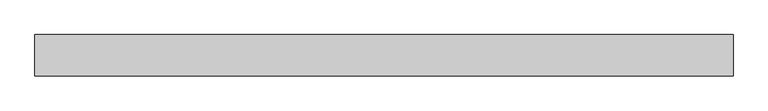
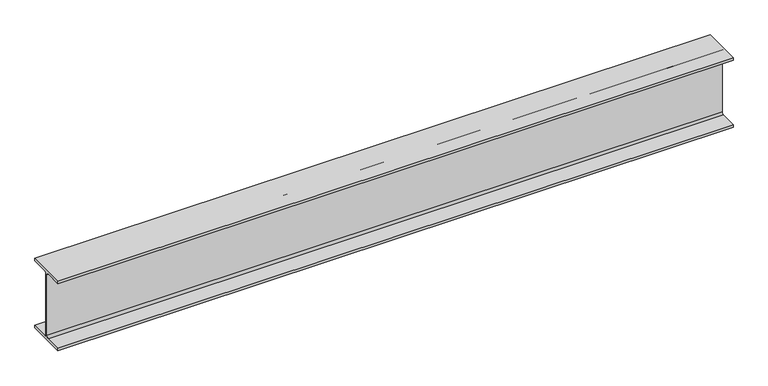
"""IFC4 building model written with IfcOpenShell, lengths in millimetres: beam geometry, Old_Steel Beam_H-KSD3502 : H_SB_ASB_H-250×125x6x9."""

import ifcopenshell
import ifcopenshell.guid

model = None  # the IFC model being written
_history = None  # IfcOwnerHistory: only IFC2X3 demands one
_inside = {}  # id of a spatial element -> (the spatial element, [elements in it])
_under = {}  # id of a project, library or spatial element -> (it, [spatial elements below it])
_declared = {}  # id of a project -> (the project, [libraries it declares])
_typed = {}  # id of a type object -> (the type object, [elements of that type])
_made_of = {}  # id of a material, layer set ... -> (it, [elements and type objects made of it])


def new_model(schema):
    """Start an empty IFC model of exactly this schema.

    Asked for "IFC4X3", IfcOpenShell would pick the latest addendum, in which some entities
    have other attributes; the version numbers below select the first issue.
    IFC2X3 requires an IfcOwnerHistory on every rooted entity: one is made here for all.
    """
    global model, _history
    if schema == "IFC4X3":
        model = ifcopenshell.file(schema_version=(4, 3, 0, 0))
    else:
        model = ifcopenshell.file(schema=schema)
    _inside.clear()
    _under.clear()
    _declared.clear()
    _typed.clear()
    _made_of.clear()
    _history = None
    if model.schema == "IFC2X3":
        org = make("IfcOrganization", Name="unknown")
        user = make(
            "IfcPersonAndOrganization",
            ThePerson=make("IfcPerson", FamilyName="unknown"),
            TheOrganization=org,
        )
        app = make(
            "IfcApplication",
            ApplicationDeveloper=org,
            Version="unknown",
            ApplicationFullName="unknown",
            ApplicationIdentifier="unknown",
        )
        _history = make(
            "IfcOwnerHistory",
            OwningUser=user,
            OwningApplication=app,
            ChangeAction="ADDED",
            CreationDate=0,
        )
    return model


def make(cls, **values):
    """One entity of the class cls with the attributes given. An attribute that is None is left unset."""
    return model.create_entity(
        cls, **{name: value for name, value in values.items() if value is not None}
    )


def rooted(cls, **values):
    """An entity with a GlobalId (a new one), such as an element, a storey or a relation."""
    return make(cls, GlobalId=ifcopenshell.guid.new(), OwnerHistory=_history, **values)


def si_unit(unit_type, name, prefix=None):
    """IfcSIUnit, for example si_unit("LENGTHUNIT", "METRE", prefix="MILLI")."""
    return make("IfcSIUnit", UnitType=unit_type, Prefix=prefix, Name=name)


def assignment(units):
    """IfcUnitAssignment: the units of a project."""
    return None if units is None else make("IfcUnitAssignment", Units=units)


def point(xyz):
    """IfcCartesianPoint."""
    return None if xyz is None else make("IfcCartesianPoint", Coordinates=xyz)


def direction(xyz):
    """IfcDirection."""
    return None if xyz is None else make("IfcDirection", DirectionRatios=xyz)


def frame(location, z_axis=None, x_axis=None):
    """IfcAxis2Placement3D, a coordinate frame: its origin and axes. An axis left out is left unset."""
    return make(
        "IfcAxis2Placement3D",
        Location=point(location),
        Axis=direction(z_axis),
        RefDirection=direction(x_axis),
    )


def frame_2d(location, x_axis=None):
    """IfcAxis2Placement2D, a coordinate frame in the plane: its origin and x axis."""
    return make(
        "IfcAxis2Placement2D", Location=point(location), RefDirection=direction(x_axis)
    )


def origin():
    """The frame at (0, 0, 0) with its axes left unset."""
    return frame((0.0, 0.0, 0.0))


def place(relative_to, where):
    """IfcLocalPlacement: puts the frame where relative to a parent placement (None: the world)."""
    return make(
        "IfcLocalPlacement", PlacementRelTo=relative_to, RelativePlacement=where
    )


def context(
    kind, dimensions, precision=None, world=None, true_north=None, identifier=None
):
    """IfcGeometricRepresentationContext, for example the 3D "Model" context."""
    return make(
        "IfcGeometricRepresentationContext",
        ContextIdentifier=identifier,
        ContextType=kind,
        CoordinateSpaceDimension=dimensions,
        Precision=precision,
        WorldCoordinateSystem=world,
        TrueNorth=true_north,
    )


def project(units=None, contexts=None):
    """IfcProject with its units and contexts."""
    return rooted(
        "IfcProject",
        Name="project",
        RepresentationContexts=contexts,
        UnitsInContext=assignment(units),
    )


def spatial(cls, under=None, at=None, **own):
    """A site, building, storey or space (cls), placed at a placement, below another one or the project."""
    s = rooted(cls, ObjectPlacement=at, **own)
    if under is not None:
        _under.setdefault(under.id(), (under, []))[1].append(s)
    return s


def polyline(points):
    """IfcPolyline through the points."""
    return make("IfcPolyline", Points=[point(p) for p in points])


def circle_curve(where, radius):
    """IfcCircle in the frame where."""
    return make("IfcCircle", Position=where, Radius=radius)


def trimmed(basis, trim1, trim2, sense, master):
    """IfcTrimmedCurve: the piece of a basis curve between two trims."""
    return make(
        "IfcTrimmedCurve",
        BasisCurve=basis,
        Trim1=trim1,
        Trim2=trim2,
        SenseAgreement=sense,
        MasterRepresentation=master,
    )


def segment(curve, same_sense, transition):
    """IfcCompositeCurveSegment."""
    return make(
        "IfcCompositeCurveSegment",
        Transition=transition,
        SameSense=same_sense,
        ParentCurve=curve,
    )


def composite_curve(segments, self_intersect=None):
    """IfcCompositeCurve: segments joined end to end."""
    return make("IfcCompositeCurve", Segments=segments, SelfIntersect=self_intersect)


def outline(outer, holes=None, kind="AREA"):
    """IfcArbitraryClosedProfileDef: a profile drawn as a closed curve; with holes, ...WithVoids."""
    if holes is None:
        return make("IfcArbitraryClosedProfileDef", ProfileType=kind, OuterCurve=outer)
    return make(
        "IfcArbitraryProfileDefWithVoids",
        ProfileType=kind,
        OuterCurve=outer,
        InnerCurves=holes,
    )


def extrude(swept, where, along, depth):
    """IfcExtrudedAreaSolid: the profile swept, set in the frame where, extruded along a direction by depth."""
    return make(
        "IfcExtrudedAreaSolid",
        SweptArea=swept,
        Position=where,
        ExtrudedDirection=direction(along),
        Depth=depth,
    )


def shape(context_of_items, identifier, shape_type, items):
    """IfcShapeRepresentation: the items that make up one representation, for example the "Body"."""
    return make(
        "IfcShapeRepresentation",
        ContextOfItems=context_of_items,
        RepresentationIdentifier=identifier,
        RepresentationType=shape_type,
        Items=items,
    )


def source(mapping_origin, context_of_items, identifier, shape_type, items):
    """IfcRepresentationMap: a shape defined once, which mapped items show again and again."""
    return make(
        "IfcRepresentationMap",
        MappingOrigin=mapping_origin,
        MappedRepresentation=shape(context_of_items, identifier, shape_type, items),
    )


def transform(
    local_origin,
    x_axis=None,
    y_axis=None,
    z_axis=None,
    scale=None,
    scale2=None,
    scale3=None,
    uniform=True,
):
    """IfcCartesianTransformationOperator3D, or its non-uniform kind. x_axis, y_axis, z_axis: its Axis1, 2, 3."""
    if uniform:
        return make(
            "IfcCartesianTransformationOperator3D",
            Axis1=direction(x_axis),
            Axis2=direction(y_axis),
            LocalOrigin=point(local_origin),
            Scale=scale,
            Axis3=direction(z_axis),
        )
    return make(
        "IfcCartesianTransformationOperator3DnonUniform",
        Axis1=direction(x_axis),
        Axis2=direction(y_axis),
        LocalOrigin=point(local_origin),
        Scale=scale,
        Axis3=direction(z_axis),
        Scale2=scale2,
        Scale3=scale3,
    )


def mapped(mapping_source, mapping_target):
    """IfcMappedItem: shows the shape of a source again, moved by a transform."""
    return make(
        "IfcMappedItem", MappingSource=mapping_source, MappingTarget=mapping_target
    )


def made_of(thing, what):
    """Note that an element or type object is made of a material, layer set ...; save() writes the relation."""
    if what is not None:
        _made_of.setdefault(what.id(), (what, []))[1].append(thing)
    return thing


def element(
    cls,
    number,
    at=None,
    inside=None,
    cuts=None,
    type_object=None,
    material=None,
    context=None,
    identifier="Body",
    shape_type=None,
    held_by="IfcProductDefinitionShape",
    body=None,
    shapes=None,
    **own,
):
    """One element of the class cls, such as IfcWall. Its Tag is "e" and its number.

    at: its placement. inside: the storey or other place that contains it. cuts: it is an
    opening in that element (IfcRelVoidsElement). A single representation is given by context,
    identifier, shape_type and body (its items); several are given by shapes. held_by: the class
    of the entity that holds the representations. save() writes the other relations.
    """
    e = rooted(cls, Tag="e%d" % number, ObjectPlacement=at, **own)
    if body is not None:
        shapes = [shape(context, identifier, shape_type, body)]
    if shapes is not None:
        e.Representation = make(held_by, Representations=shapes)
    if inside is not None:
        _inside.setdefault(inside.id(), (inside, []))[1].append(e)
    if cuts is not None:
        rooted(
            "IfcRelVoidsElement", RelatingBuildingElement=cuts, RelatedOpeningElement=e
        )
    if type_object is not None:
        _typed.setdefault(type_object.id(), (type_object, []))[1].append(e)
    return made_of(e, material)


def aggregate(whole, parts):
    """IfcRelAggregates: a whole, such as a stair, and the parts it consists of."""
    return rooted("IfcRelAggregates", RelatingObject=whole, RelatedObjects=parts)


def save(model, path):
    """Write the relations noted so far, then the file.

    IfcRelAggregates (storeys below a building ...), IfcRelContainedInSpatialStructure (elements
    in a storey), IfcRelDefinesByType, IfcRelAssociatesMaterial and IfcRelDeclares: one each for
    every whole, place, type object, material and project.
    """
    for whole, parts in _under.values():
        aggregate(whole, parts)
    for where, things in _inside.values():
        rooted(
            "IfcRelContainedInSpatialStructure",
            RelatedElements=things,
            RelatingStructure=where,
        )
    for kind, things in _typed.values():
        rooted("IfcRelDefinesByType", RelatedObjects=things, RelatingType=kind)
    for what, things in _made_of.values():
        rooted("IfcRelAssociatesMaterial", RelatedObjects=things, RelatingMaterial=what)
    for by, libraries in _declared.values():
        rooted("IfcRelDeclares", RelatingContext=by, RelatedDefinitions=libraries)
    model.write(path)


def beam_b824a9ea(model_context):
    return source(origin(), model_context, "Body", "SweptSolid", [
        extrude(outline(composite_curve([segment(polyline([(82.5, -141.5), (82.5, -151.7), (-82.5, -151.7), (-82.5, -141.5), (-11.9, -141.5)]), True, "CONTINUOUS"), segment(trimmed(circle_curve(frame_2d((-11.9, -132.6)), 8.9), [point((-11.9, -141.5))], [point((-3.0, -132.6))], True, "CARTESIAN"), True, "CONTINUOUS"), segment(polyline([(-3.0, -132.6), (-3.0, 132.6)]), True, "CONTINUOUS"), segment(trimmed(circle_curve(frame_2d((-11.9, 132.6)), 8.9), [point((-3.0, 132.6))], [point((-11.9, 141.5))], True, "CARTESIAN"), True, "CONTINUOUS"), segment(polyline([(-11.9, 141.5), (-82.5, 141.5), (-82.5, 151.7), (82.5, 151.7), (82.5, 141.5), (11.9, 141.5)]), True, "CONTINUOUS"), segment(trimmed(circle_curve(frame_2d((11.9, 132.6)), 8.9), [point((11.9, 141.5))], [point((3.0, 132.6))], True, "CARTESIAN"), True, "CONTINUOUS"), segment(polyline([(3.0, 132.6), (3.0, -132.6)]), True, "CONTINUOUS"), segment(trimmed(circle_curve(frame_2d((11.9, -132.6)), 8.9), [point((3.0, -132.6))], [point((11.9, -141.5))], True, "CARTESIAN"), True, "CONTINUOUS"), segment(polyline([(11.9, -141.5), (82.5, -141.5)]), True, "CONTINUOUS")], self_intersect=False)), frame((-1382.2982577, 0.0, 0.0), z_axis=(1.0, 0.0, 0.0), x_axis=(0.0, 1.0, 0.0)), (0.0, 0.0, 1.0), 2794.5982507),
    ])


if __name__ == "__main__":
    model = new_model("IFC4")
    model_context = context("Model", 3, world=origin())
    ifc_project = project(units=[si_unit("LENGTHUNIT", "METRE", prefix="MILLI")], contexts=[model_context])
    site = spatial("IfcSite", under=ifc_project)
    building = spatial("IfcBuilding", under=site)
    placement = place(None, origin())
    beam_shape = beam_b824a9ea(model_context)
    element("IfcBeam", 1, ObjectType="Old_Steel Beam_H-KSD3502 : H_SB_ASB_H-250×125x6x9", at=placement, inside=building, context=model_context, shape_type="MappedRepresentation", body=[
        mapped(beam_shape, transform((0.0, 0.0, 0.0), x_axis=(1.0, 0.0, 0.0), y_axis=(0.0, 1.0, 0.0), z_axis=(0.0, 0.0, 1.0))),
    ])
    save(model, "model.ifc")

# Revit data of these elements
# Type "Old_Steel Beam_H-KSD3502 : H_SB_ASB_H-250×125x6x9"
#   Width = 12.5 cm
#   Web Thickness = 0.6 cm
#   Web Fillet = 1.2 cm
#   Warping Constant = 42539.8 cm⁶
#   Torsional Moment of Inertia = 7.8102 cm⁴
#   Torsional Modulus = 1.0 cm³
#   Section Area = 37.66 cm²
#   Plastic Modulus weak axis = 73.1 cm³
#   Plastic Modulus strong axis = 366.0 cm³
#   Perimeter = 0.97 m²/m
#   Nominal Weight = 29.60 kgf/m
#   Moment of Inertia weak axis = 294.00 cm⁴
#   Moment of Inertia strong axis = 4050.00 cm⁴
#   Height = 25.0 cm
#   Flange Thickness = 0.9 cm
#   Elastic Modulus weak axis = 47.0 cm³
#   Elastic Modulus strong axis = 324.0 cm³
#   Centroid Vertical = 12.5 cm
#   Centroid Horizontal = 6.25 cm
#   Length [instance default] = 1.5240 m
#   Structural Material [instance default] = Steel, 45-345
#   Assembly Code = ""
# Element 1 (IfcBeam, "Old_Steel Beam_H-KSD3502 : H_SB_ASB_H-250×125x6x9")
#   Structural Material = none
# Materials
#   "Steel, 45-345": class "Metal", colour RGB 189 187 185, transparency 0, Description = "Steel 345 MPa", Cost = 0
